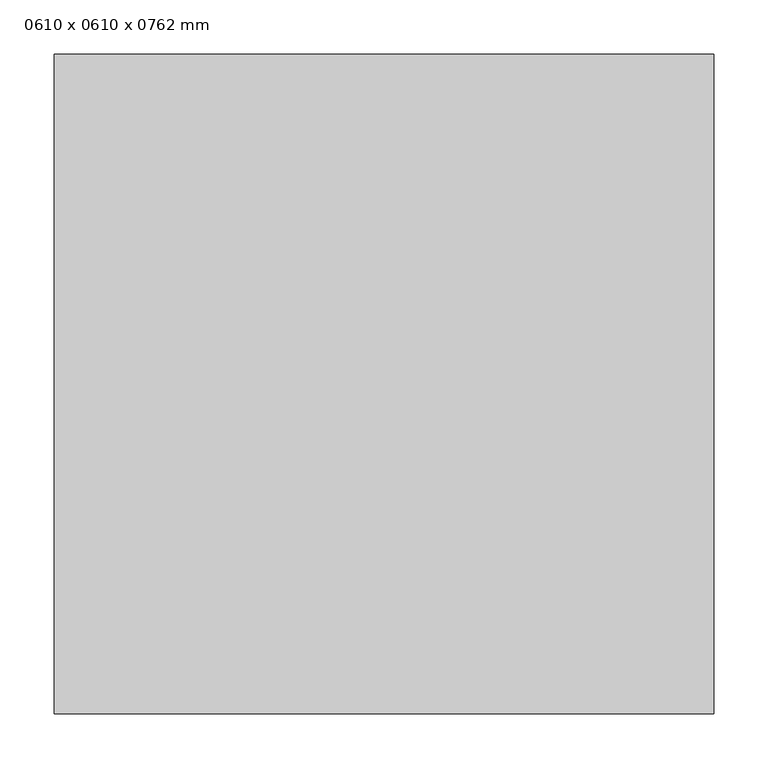
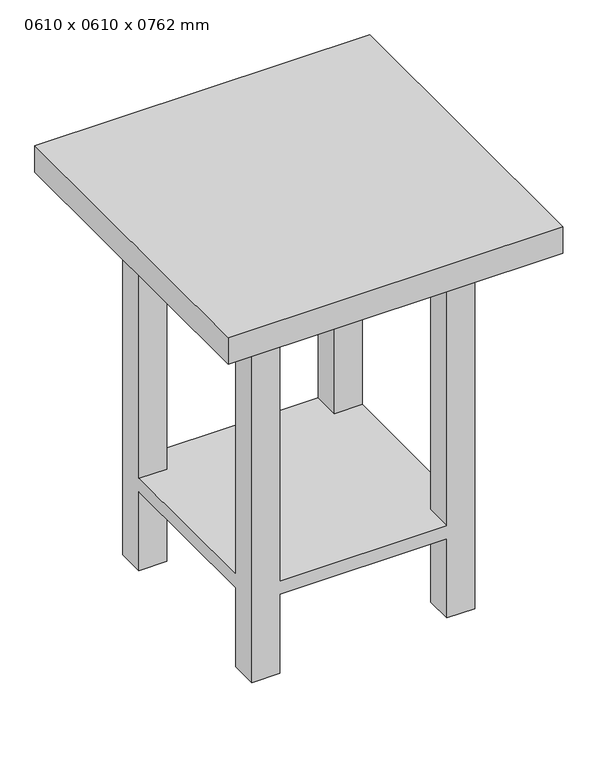
"""IFC4 building model written with IfcOpenShell, lengths in millimetres: furniture geometry, Mesa-Mesita de noche : 0610 x 0610 x 0762 mm."""

from ifc_helpers import new_model, si_unit, frame, origin, place, context, project, spatial, polyline, outline, extrude, faceted_brep, source, transform, mapped, element, save


def furniture_0610_x_0610_x_0762_mm_52c223ea(model_context):
    return source(origin(), model_context, "Body", "SolidModel", [
        faceted_brep([(156.1336303, -508.4, 711.2), (156.1336303, -457.6, 711.2), (105.3336303, -457.6, 711.2), (105.3336303, -508.4, 711.2), (156.1336303, -152.4, 711.2), (156.1336303, -101.6, 711.2), (105.3336303, -101.6, 711.2), (105.3336303, -152.4, 711.2), (512.1336303, -508.4, 711.2), (512.1336303, -457.6, 711.2), (461.3336303, -457.6, 711.2), (461.3336303, -508.4, 711.2), (512.1336303, -152.4, 711.2), (512.1336303, -101.6, 711.2), (461.3336303, -101.6, 711.2), (461.3336303, -152.4, 711.2), (156.1336303, -508.4, 0.0), (105.3336303, -508.4, 0.0), (105.3336303, -457.6, 0.0), (156.1336303, -457.6, 0.0), (156.1336303, -152.4, 0.0), (105.3336303, -152.4, 0.0), (105.3336303, -101.6, 0.0), (156.1336303, -101.6, 0.0), (512.1336303, -508.4, 0.0), (461.3336303, -508.4, 0.0), (461.3336303, -457.6, 0.0), (512.1336303, -457.6, 0.0), (512.1336303, -152.4, 0.0), (461.3336303, -152.4, 0.0), (461.3336303, -101.6, 0.0), (512.1336303, -101.6, 0.0), (156.1336303, -508.4, 152.4), (461.3336303, -508.4, 152.4), (461.3336303, -508.4, 177.8), (156.1336303, -508.4, 177.8), (105.3336303, -457.6, 177.8), (105.3336303, -152.4, 177.8), (105.3336303, -152.4, 152.4), (105.3336303, -457.6, 152.4), (156.1336303, -457.6, 152.4), (156.1336303, -457.6, 177.8), (156.1336303, -152.4, 177.8), (156.1336303, -152.4, 152.4), (156.1336303, -101.6, 177.8), (461.3336303, -101.6, 177.8), (461.3336303, -101.6, 152.4), (156.1336303, -101.6, 152.4), (461.3336303, -457.6, 152.4), (461.3336303, -457.6, 177.8), (512.1336303, -457.6, 152.4), (512.1336303, -457.6, 177.8), (512.1336303, -152.4, 152.4), (512.1336303, -152.4, 177.8), (461.3336303, -152.4, 152.4), (461.3336303, -152.4, 177.8)], [[[0, 1, 2, 3]], [[4, 5, 6, 7]], [[8, 9, 10, 11]], [[12, 13, 14, 15]], [[16, 17, 18, 19]], [[20, 21, 22, 23]], [[24, 25, 26, 27]], [[28, 29, 30, 31]], [[3, 17, 16, 32, 33, 25, 24, 8, 11, 34, 35, 0]], [[2, 36, 37, 7, 6, 22, 21, 38, 39, 18, 17, 3]], [[18, 39, 40, 19]], [[1, 41, 36, 2]], [[0, 35, 41, 1]], [[19, 40, 32, 16]], [[7, 37, 42, 4]], [[20, 43, 38, 21]], [[5, 44, 45, 14, 13, 31, 30, 46, 47, 23, 22, 6]], [[4, 42, 44, 5]], [[23, 47, 43, 20]], [[25, 33, 48, 26]], [[10, 49, 34, 11]], [[26, 48, 50, 27]], [[9, 51, 49, 10]], [[8, 24, 27, 50, 52, 28, 31, 13, 12, 53, 51, 9]], [[28, 52, 54, 29]], [[15, 55, 53, 12]], [[14, 45, 55, 15]], [[29, 54, 46, 30]], [[36, 41, 35, 34, 49, 51, 53, 55, 45, 44, 42, 37]], [[32, 40, 39, 38, 43, 47, 46, 54, 52, 50, 48, 33]]]),
        extrude(outline(polyline([(613.7336303, 0.0), (613.7336303, -610.0), (3.7336303, -610.0), (3.7336303, 0.0), (613.7336303, 0.0)])), frame((0.0, 0.0, 711.2), z_axis=(0.0, 0.0, 1.0), x_axis=(1.0, 0.0, 0.0)), (0.0, 0.0, 1.0), 50.8),
    ])


if __name__ == "__main__":
    model = new_model("IFC4")
    model_context = context("Model", 3, world=origin())
    ifc_project = project(units=[si_unit("LENGTHUNIT", "METRE", prefix="MILLI")], contexts=[model_context])
    site = spatial("IfcSite", under=ifc_project)
    building = spatial("IfcBuilding", under=site)
    placement = place(None, origin())
    furniture_0610_x_0610_x_0762_mm_shape = furniture_0610_x_0610_x_0762_mm_52c223ea(model_context)
    element("IfcFurniture", 1, ObjectType="Mesa-Mesita de noche : 0610 x 0610 x 0762 mm", at=placement, inside=building, context=model_context, shape_type="MappedRepresentation", body=[
        mapped(furniture_0610_x_0610_x_0762_mm_shape, transform((0.0, 0.0, 0.0), x_axis=(1.0, 0.0, 0.0), y_axis=(0.0, 1.0, 0.0), z_axis=(0.0, 0.0, 1.0))),
    ])
    save(model, "model.ifc")

# Revit data of these elements
# Type "Mesa-Mesita de noche : 0610 x 0610 x 0762 mm"
#   Profundidad = 0.61 m
#   Altura = 0.762 m
#   Anchura = 0.61 m
#   Máscara [instance default] = yes
#   Material base = Madera - Abedul
#   Material de parte superior = Laminado - Marfil, Mate
#   Default Elevation = 0
# Element 1 (IfcFurniture, "Mesa-Mesita de noche : 0610 x 0610 x 0762 mm")
#   Materials on its faces: "Madera - Abedul", "Laminado - Marfil, Mate"
# Materials
#   "Madera - Abedul": class "Madera", colour RGB 224 178 126, transparency 0
#   "Laminado - Marfil, Mate": class "Varios", colour RGB 247 247 239, transparency 0
